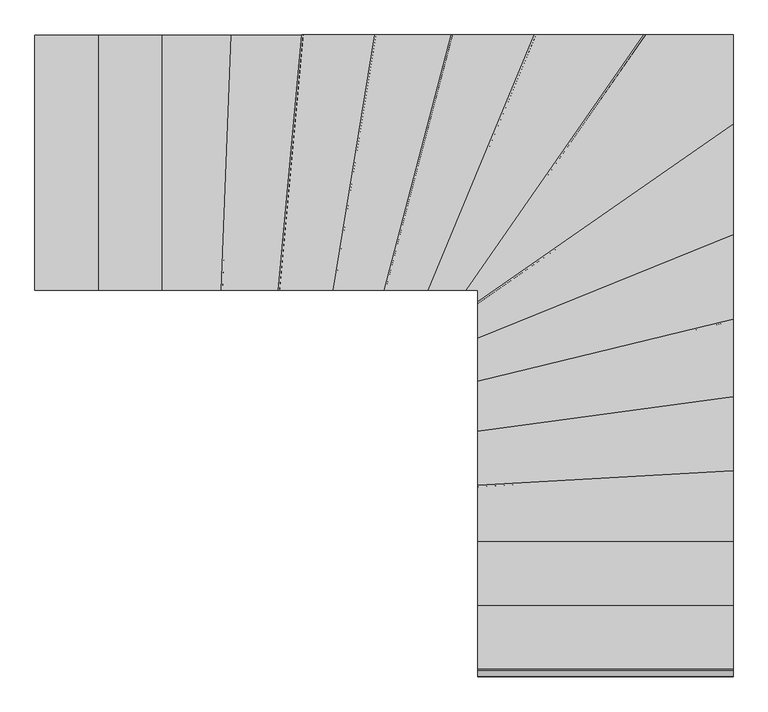
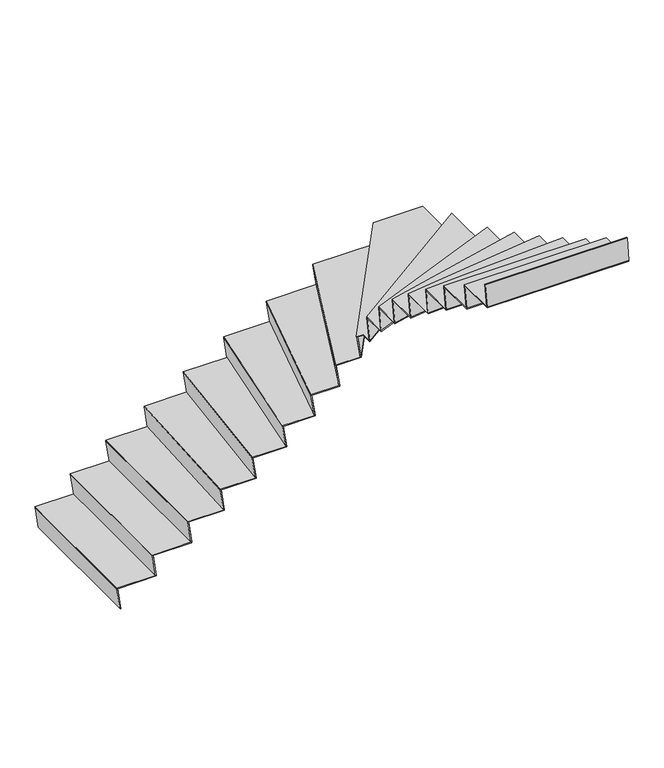
"""IFC4 building model written with IfcOpenShell, lengths in millimetres: stair flight geometry."""

from ifc_helpers import new_model, si_unit, origin, place, context, project, spatial, faceted_brep, source, transform, mapped, element, save


def stair_flight_e103a2b8(model_context):
    return source(origin(), model_context, "Body", "Brep", [
        faceted_brep([(2065.7472679, 3026.6218979, 176.4705882), (2066.5972679, 3026.6218979, 170.4705882), (2066.5972679, 4126.6218979, 170.4705882), (2065.7472679, 4126.6218979, 176.4705882), (1759.6873587, 4126.6218979, 176.4705882), (1759.6873587, 3026.6218979, 176.4705882), (1760.5373587, 3026.6218979, 170.4705882), (1760.5373587, 4126.6218979, 170.4705882)], [[[0, 1, 2, 3]], [[3, 4, 5, 0]], [[2, 1, 6, 7]], [[4, 3, 2, 7]], [[0, 5, 6, 1]], [[5, 4, 7, 6]]]),
        faceted_brep([(1760.5373587, 3026.6218979, 170.4705882), (1784.6873587, 3026.6218979, 0.0), (1790.7472679, 3026.6218979, 0.0), (1766.5972679, 3026.6218979, 170.4705882), (1760.5373587, 4126.6218979, 170.4705882), (1766.5972679, 4126.6218979, 170.4705882), (1790.7472679, 4126.6218979, 0.0), (1784.6873587, 4126.6218979, 0.0)], [[[0, 1, 2, 3]], [[4, 5, 6, 7]], [[1, 0, 4, 7]], [[2, 1, 7, 6]], [[3, 2, 6, 5]], [[0, 3, 5, 4]]]),
        faceted_brep([(2035.5373587, 3026.6218979, 346.9411765), (2059.6873587, 3026.6218979, 176.4705882), (2065.7472679, 3026.6218979, 176.4705882), (2041.5972679, 3026.6218979, 346.9411765), (2035.5373587, 4126.6218979, 346.9411765), (2041.5972679, 4126.6218979, 346.9411765), (2065.7472679, 4126.6218979, 176.4705882), (2059.6873587, 4126.6218979, 176.4705882)], [[[0, 1, 2, 3]], [[4, 5, 6, 7]], [[1, 0, 4, 7]], [[2, 1, 7, 6]], [[3, 2, 6, 5]], [[0, 3, 5, 4]]]),
        faceted_brep([(2340.7472679, 4126.6218979, 352.9411765), (2034.6873587, 4126.6218979, 352.9411765), (2034.6873587, 3026.6218979, 352.9411765), (2340.7472679, 3026.6218979, 352.9411765), (2341.5972679, 4126.6218979, 346.9411765), (2341.5972679, 3026.6218979, 346.9411765), (2035.5373587, 3026.6218979, 346.9411765), (2035.5373587, 4126.6218979, 346.9411765)], [[[0, 1, 2, 3]], [[4, 5, 6, 7]], [[1, 0, 4, 7]], [[3, 2, 6, 5]], [[3, 5, 4, 0]], [[2, 1, 7, 6]]]),
        faceted_brep([(2310.5373587, 3026.6218979, 523.4117647), (2334.6873587, 3026.6218979, 352.9411765), (2340.7472679, 3026.6218979, 352.9411765), (2316.5972679, 3026.6218979, 523.4117647), (2310.5373587, 4126.6218979, 523.4117647), (2316.5972679, 4126.6218979, 523.4117647), (2340.7472679, 4126.6218979, 352.9411765), (2334.6873587, 4126.6218979, 352.9411765)], [[[0, 1, 2, 3]], [[4, 5, 6, 7]], [[1, 0, 4, 7]], [[2, 1, 7, 6]], [[3, 2, 6, 5]], [[0, 3, 5, 4]]]),
        faceted_brep([(2637.9370393, 4126.6218979, 529.4117647), (2309.6873587, 4126.6218979, 529.4117647), (2309.6873587, 3026.6218979, 529.4117647), (2593.6079182, 3026.6218979, 529.4117647), (2638.7877292, 4126.6218979, 523.4117647), (2594.4586082, 3026.6218979, 523.4117647), (2310.5373587, 3026.6218979, 523.4117647), (2310.5373587, 4126.6218979, 523.4117647)], [[[0, 1, 2, 3]], [[4, 5, 6, 7]], [[1, 0, 4, 7]], [[3, 2, 6, 5]], [[3, 5, 4, 0]], [[2, 1, 7, 6]]]),
        faceted_brep([(2563.3734881, 3026.6218979, 699.8823529), (2587.5430903, 3026.6218979, 529.4117647), (2593.6079182, 3026.6218979, 529.4117647), (2569.4383161, 3026.6218979, 699.8823529), (2607.7026092, 4126.6218979, 699.8823529), (2613.7674371, 4126.6218979, 699.8823529), (2637.9370393, 4126.6218979, 529.4117647), (2631.8722113, 4126.6218979, 529.4117647)], [[[0, 1, 2, 3]], [[4, 5, 6, 7]], [[1, 0, 4, 7]], [[2, 1, 7, 6]], [[3, 2, 6, 5]], [[0, 3, 5, 4]]]),
        faceted_brep([(2941.764971, 4126.6218979, 705.8823529), (2606.8519192, 4126.6218979, 705.8823529), (2562.5227982, 3026.6218979, 705.8823529), (2839.9948598, 3026.6218979, 705.8823529), (2942.6186011, 4126.6218979, 699.8823529), (2840.8484899, 3026.6218979, 699.8823529), (2563.3734881, 3026.6218979, 699.8823529), (2607.7026092, 4126.6218979, 699.8823529)], [[[0, 1, 2, 3]], [[4, 5, 6, 7]], [[1, 0, 4, 7]], [[3, 2, 6, 5]], [[3, 5, 4, 0]], [[2, 1, 7, 6]]]),
        faceted_brep([(2809.6559332, 3026.6218979, 876.3529412), (2833.9090705, 3026.6218979, 705.8823529), (2839.9948598, 3026.6218979, 705.8823529), (2815.7417225, 3026.6218979, 876.3529412), (2911.4260444, 4126.6218979, 876.3529412), (2917.5118337, 4126.6218979, 876.3529412), (2941.764971, 4126.6218979, 705.8823529), (2935.6791818, 4126.6218979, 705.8823529)], [[[0, 1, 2, 3]], [[4, 5, 6, 7]], [[1, 0, 4, 7]], [[2, 1, 7, 6]], [[3, 2, 6, 5]], [[0, 3, 5, 4]]]),
        faceted_brep([(3255.7315376, 4126.6218979, 882.3529412), (2910.5724143, 4126.6218979, 882.3529412), (2808.8023031, 3026.6218979, 882.3529412), (3076.5814578, 3026.6218979, 882.3529412), (3256.5927368, 4126.6218979, 876.3529412), (3077.442657, 3026.6218979, 876.3529412), (2809.6559332, 3026.6218979, 876.3529412), (2911.4260444, 4126.6218979, 876.3529412)], [[[0, 1, 2, 3]], [[4, 5, 6, 7]], [[1, 0, 4, 7]], [[3, 2, 6, 5]], [[3, 5, 4, 0]], [[2, 1, 7, 6]]]),
        faceted_brep([(3045.973518, 3026.6218979, 1052.8235294), (3070.4417062, 3026.6218979, 882.3529412), (3076.5814578, 3026.6218979, 882.3529412), (3052.1132695, 3026.6218979, 1052.8235294), (3225.1235978, 4126.6218979, 1052.8235294), (3231.2633493, 4126.6218979, 1052.8235294), (3255.7315376, 4126.6218979, 882.3529412), (3249.591786, 4126.6218979, 882.3529412)], [[[0, 1, 2, 3]], [[4, 5, 6, 7]], [[1, 0, 4, 7]], [[2, 1, 7, 6]], [[3, 2, 6, 5]], [[0, 3, 5, 4]]]),
        faceted_brep([(3586.3171605, 4126.6218979, 1058.8235294), (3224.2623986, 4126.6218979, 1058.8235294), (3045.1123188, 3026.6218979, 1058.8235294), (3297.2859801, 3026.6218979, 1058.8235294), (3587.196013, 4126.6218979, 1052.8235294), (3298.1648327, 3026.6218979, 1052.8235294), (3045.973518, 3026.6218979, 1052.8235294), (3225.1235978, 4126.6218979, 1052.8235294)], [[[0, 1, 2, 3]], [[4, 5, 6, 7]], [[1, 0, 4, 7]], [[3, 2, 6, 5]], [[3, 5, 4, 0]], [[2, 1, 7, 6]]]),
        faceted_brep([(3266.0506211, 3026.6218979, 1229.2941176), (3291.0203724, 3026.6218979, 1058.8235294), (3297.2859801, 3026.6218979, 1058.8235294), (3272.3162288, 3026.6218979, 1229.2941176), (3555.0818014, 4126.6218979, 1229.2941176), (3561.3474091, 4126.6218979, 1229.2941176), (3586.3171605, 4126.6218979, 1058.8235294), (3580.0515527, 4126.6218979, 1058.8235294)], [[[0, 1, 2, 3]], [[4, 5, 6, 7]], [[1, 0, 4, 7]], [[2, 1, 7, 6]], [[3, 2, 6, 5]], [[0, 3, 5, 4]]]),
        faceted_brep([(3947.0915643, 4126.6218979, 1235.2941176), (3554.2029489, 4126.6218979, 1235.2941176), (3265.1717685, 3026.6218979, 1235.2941176), (3489.7295318, 3026.6218979, 1235.2941176), (3948.0121092, 4126.6218979, 1229.2941176), (3490.6500767, 3026.6218979, 1229.2941176), (3266.0506211, 3026.6218979, 1229.2941176), (3555.0818014, 4126.6218979, 1229.2941176)], [[[0, 1, 2, 3]], [[4, 5, 6, 7]], [[1, 0, 4, 7]], [[3, 2, 6, 5]], [[3, 5, 4, 0]], [[2, 1, 7, 6]]]),
        faceted_brep([(3457.0123806, 3026.6218979, 1405.7647059), (3483.1666863, 3026.6218979, 1235.2941176), (3489.7295318, 3026.6218979, 1235.2941176), (3463.5752261, 3026.6218979, 1405.7647059), (3914.3744131, 4126.6218979, 1405.7647059), (3920.9372586, 4126.6218979, 1405.7647059), (3947.0915643, 4126.6218979, 1235.2941176), (3940.5287188, 4126.6218979, 1235.2941176)], [[[0, 1, 2, 3]], [[4, 5, 6, 7]], [[1, 0, 4, 7]], [[2, 1, 7, 6]], [[3, 2, 6, 5]], [[0, 3, 5, 4]]]),
        faceted_brep([(4423.3254739, 4126.6218979, 1411.7647059), (3913.4538681, 4126.6218979, 1411.7647059), (3456.0918357, 3026.6218979, 1411.7647059), (3656.5915421, 3026.6218979, 1411.7647059), (4424.3615859, 4126.6218979, 1405.7647059), (3657.6276541, 3026.6218979, 1405.7647059), (3457.0123806, 3026.6218979, 1405.7647059), (3914.3744131, 4126.6218979, 1405.7647059)], [[[0, 1, 2, 3]], [[4, 5, 6, 7]], [[1, 0, 4, 7]], [[3, 2, 6, 5]], [[3, 5, 4, 0]], [[2, 1, 7, 6]]]),
        faceted_brep([(3619.7670134, 3026.6218979, 1582.2352941), (3649.2047837, 3026.6218979, 1411.7647059), (3656.5915421, 3026.6218979, 1411.7647059), (3627.1537718, 3026.6218979, 1582.2352941), (4386.5009452, 4126.6218979, 1582.2352941), (4393.8877036, 4126.6218979, 1582.2352941), (4423.3254739, 4126.6218979, 1411.7647059), (4415.9387155, 4126.6218979, 1411.7647059)], [[[0, 1, 2, 3]], [[4, 5, 6, 7]], [[1, 0, 4, 7]], [[2, 1, 7, 6]], [[3, 2, 6, 5]], [[0, 3, 5, 4]]]),
        faceted_brep([(4769.6425896, 3704.5835008, 1588.2352941), (4769.6425896, 4126.6218979, 1588.2352941), (4385.4648332, 4126.6218979, 1588.2352941), (3618.7309014, 3026.6218979, 1588.2352941), (3669.6425896, 3026.6218979, 1588.2352941), (3669.6425896, 2937.849569, 1588.2352941), (4769.6425896, 3703.5473888, 1582.2352941), (3669.6425896, 2936.813457, 1582.2352941), (3669.6425896, 3026.6218979, 1582.2352941), (3619.7670134, 3026.6218979, 1582.2352941), (4386.5009452, 4126.6218979, 1582.2352941), (4769.6425896, 4126.6218979, 1582.2352941)], [[[0, 1, 2, 3, 4, 5]], [[6, 7, 8, 9, 10, 11]], [[1, 0, 6, 11]], [[2, 1, 11, 10]], [[4, 3, 9, 8]], [[5, 4, 8, 7]], [[5, 7, 6, 0]], [[3, 2, 10, 9]]]),
        faceted_brep([(3669.6425896, 2974.6740977, 1758.7058824), (3669.6425896, 2945.2363274, 1588.2352941), (3669.6425896, 2937.849569, 1588.2352941), (3669.6425896, 2967.2873392, 1758.7058824), (4769.6425896, 3741.4080295, 1758.7058824), (4769.6425896, 3734.0212711, 1758.7058824), (4769.6425896, 3704.5835008, 1588.2352941), (4769.6425896, 3711.9702592, 1588.2352941)], [[[0, 1, 2, 3]], [[4, 5, 6, 7]], [[1, 0, 4, 7]], [[2, 1, 7, 6]], [[3, 2, 6, 5]], [[0, 3, 5, 4]]]),
        faceted_brep([(4769.6425896, 3231.5060834, 1764.7058824), (4769.6425896, 3742.4441415, 1764.7058824), (3669.6425896, 2975.7102097, 1764.7058824), (3669.6425896, 2784.9507322, 1764.7058824), (4769.6425896, 3230.5887121, 1758.7058824), (3669.6425896, 2784.0333608, 1758.7058824), (3669.6425896, 2974.6740977, 1758.7058824), (4769.6425896, 3741.4080295, 1758.7058824)], [[[0, 1, 2, 3]], [[4, 5, 6, 7]], [[1, 0, 4, 7]], [[3, 2, 6, 5]], [[3, 5, 4, 0]], [[2, 1, 7, 6]]]),
        faceted_brep([(3669.6425896, 2817.5550913, 1935.1764706), (3669.6425896, 2791.4909523, 1764.7058824), (3669.6425896, 2784.9507322, 1764.7058824), (3669.6425896, 2811.0148712, 1935.1764706), (4769.6425896, 3264.1104426, 1935.1764706), (4769.6425896, 3257.5702224, 1935.1764706), (4769.6425896, 3231.5060834, 1764.7058824), (4769.6425896, 3238.0463036, 1764.7058824)], [[[0, 1, 2, 3]], [[4, 5, 6, 7]], [[1, 0, 4, 7]], [[2, 1, 7, 6]], [[3, 2, 6, 5]], [[0, 3, 5, 4]]]),
        faceted_brep([(4769.6425896, 2868.6989632, 1941.1764706), (4769.6425896, 3265.027814, 1941.1764706), (3669.6425896, 2818.4724627, 1941.1764706), (3669.6425896, 2600.6974331, 1941.1764706), (4769.6425896, 2867.8240992, 1935.1764706), (3669.6425896, 2599.8225691, 1935.1764706), (3669.6425896, 2817.5550913, 1935.1764706), (4769.6425896, 3264.1104426, 1935.1764706)], [[[0, 1, 2, 3]], [[4, 5, 6, 7]], [[1, 0, 4, 7]], [[3, 2, 6, 5]], [[3, 5, 4, 0]], [[2, 1, 7, 6]]]),
        faceted_brep([(3669.6425896, 2631.7910379, 2111.6470588), (3669.6425896, 2606.9346059, 1941.1764706), (3669.6425896, 2600.6974331, 1941.1764706), (3669.6425896, 2625.5538651, 2111.6470588), (4769.6425896, 2899.792568, 2111.6470588), (4769.6425896, 2893.5553952, 2111.6470588), (4769.6425896, 2868.6989632, 1941.1764706), (4769.6425896, 2874.936136, 1941.1764706)], [[[0, 1, 2, 3]], [[4, 5, 6, 7]], [[1, 0, 4, 7]], [[2, 1, 7, 6]], [[3, 2, 6, 5]], [[0, 3, 5, 4]]]),
        faceted_brep([(4769.6425896, 2534.7846987, 2117.6470588), (4769.6425896, 2900.667432, 2117.6470588), (3669.6425896, 2632.665902, 2117.6470588), (3669.6425896, 2385.8621086, 2117.6470588), (4769.6425896, 2533.9269443, 2111.6470588), (3669.6425896, 2385.0043542, 2111.6470588), (3669.6425896, 2631.7910379, 2111.6470588), (4769.6425896, 2899.792568, 2111.6470588)], [[[0, 1, 2, 3]], [[4, 5, 6, 7]], [[1, 0, 4, 7]], [[3, 2, 6, 5]], [[3, 5, 4, 0]], [[2, 1, 7, 6]]]),
        faceted_brep([(3669.6425896, 2416.3476175, 2288.1176471), (3669.6425896, 2391.9773013, 2117.6470588), (3669.6425896, 2385.8621086, 2117.6470588), (3669.6425896, 2410.2324248, 2288.1176471), (4769.6425896, 2565.2702077, 2288.1176471), (4769.6425896, 2559.1550149, 2288.1176471), (4769.6425896, 2534.7846987, 2117.6470588), (4769.6425896, 2540.8998915, 2117.6470588)], [[[0, 1, 2, 3]], [[4, 5, 6, 7]], [[1, 0, 4, 7]], [[2, 1, 7, 6]], [[3, 2, 6, 5]], [[0, 3, 5, 4]]]),
        faceted_brep([(4769.6425896, 2217.471517, 2294.1176471), (4769.6425896, 2566.1279621, 2294.1176471), (3669.6425896, 2417.2053719, 2294.1176471), (3669.6425896, 2153.6374895, 2294.1176471), (4769.6425896, 2216.6200869, 2288.1176471), (3669.6425896, 2152.7860594, 2288.1176471), (3669.6425896, 2416.3476175, 2288.1176471), (4769.6425896, 2565.2702077, 2288.1176471)], [[[0, 1, 2, 3]], [[4, 5, 6, 7]], [[1, 0, 4, 7]], [[3, 2, 6, 5]], [[3, 5, 4, 0]], [[2, 1, 7, 6]]]),
        faceted_brep([(3669.6425896, 2183.8982232, 2464.5882353), (3669.6425896, 2159.7075938, 2294.1176471), (3669.6425896, 2153.6374895, 2294.1176471), (3669.6425896, 2177.8281189, 2464.5882353), (4769.6425896, 2247.7322507, 2464.5882353), (4769.6425896, 2241.6621464, 2464.5882353), (4769.6425896, 2217.471517, 2294.1176471), (4769.6425896, 2223.5416213, 2294.1176471)], [[[0, 1, 2, 3]], [[4, 5, 6, 7]], [[1, 0, 4, 7]], [[2, 1, 7, 6]], [[3, 2, 6, 5]], [[0, 3, 5, 4]]]),
        faceted_brep([(4769.6425896, 1910.6067578, 2470.5882353), (4769.6425896, 2248.5836807, 2470.5882353), (3669.6425896, 2184.7496533, 2470.5882353), (3669.6425896, 1910.6067578, 2470.5882353), (4769.6425896, 1909.7567578, 2464.5882353), (3669.6425896, 1909.7567578, 2464.5882353), (3669.6425896, 2183.8982232, 2464.5882353), (4769.6425896, 2247.7322507, 2464.5882353)], [[[0, 1, 2, 3]], [[4, 5, 6, 7]], [[1, 0, 4, 7]], [[3, 2, 6, 5]], [[3, 5, 4, 0]], [[2, 1, 7, 6]]]),
        faceted_brep([(3669.6425896, 1940.816667, 2641.0588235), (3669.6425896, 1916.666667, 2470.5882353), (3669.6425896, 1910.6067578, 2470.5882353), (3669.6425896, 1934.7567578, 2641.0588235), (4769.6425896, 1940.816667, 2641.0588235), (4769.6425896, 1934.7567578, 2641.0588235), (4769.6425896, 1910.6067578, 2470.5882353), (4769.6425896, 1916.666667, 2470.5882353)], [[[0, 1, 2, 3]], [[4, 5, 6, 7]], [[1, 0, 4, 7]], [[2, 1, 7, 6]], [[3, 2, 6, 5]], [[0, 3, 5, 4]]]),
        faceted_brep([(4769.6425896, 1635.6067578, 2647.0588235), (4769.6425896, 1941.666667, 2647.0588235), (3669.6425896, 1941.666667, 2647.0588235), (3669.6425896, 1635.6067578, 2647.0588235), (4769.6425896, 1634.7567578, 2641.0588235), (3669.6425896, 1634.7567578, 2641.0588235), (3669.6425896, 1940.816667, 2641.0588235), (4769.6425896, 1940.816667, 2641.0588235)], [[[0, 1, 2, 3]], [[4, 5, 6, 7]], [[1, 0, 4, 7]], [[3, 2, 6, 5]], [[3, 5, 4, 0]], [[2, 1, 7, 6]]]),
        faceted_brep([(3669.6425896, 1665.816667, 2817.5294118), (3669.6425896, 1641.666667, 2647.0588235), (3669.6425896, 1635.6067578, 2647.0588235), (3669.6425896, 1659.7567578, 2817.5294118), (4769.6425896, 1665.816667, 2817.5294118), (4769.6425896, 1659.7567578, 2817.5294118), (4769.6425896, 1635.6067578, 2647.0588235), (4769.6425896, 1641.666667, 2647.0588235)], [[[0, 1, 2, 3]], [[4, 5, 6, 7]], [[1, 0, 4, 7]], [[2, 1, 7, 6]], [[3, 2, 6, 5]], [[0, 3, 5, 4]]]),
        faceted_brep([(3669.6425896, 1390.816667, 2994.0), (3669.6425896, 1366.666667, 2823.5294118), (3669.6425896, 1360.6067578, 2823.5294118), (3669.6425896, 1384.7567578, 2994.0), (4769.6425896, 1390.816667, 2994.0), (4769.6425896, 1384.7567578, 2994.0), (4769.6425896, 1360.6067578, 2823.5294118), (4769.6425896, 1366.666667, 2823.5294118)], [[[0, 1, 2, 3]], [[4, 5, 6, 7]], [[1, 0, 4, 7]], [[2, 1, 7, 6]], [[3, 2, 6, 5]], [[0, 3, 5, 4]]]),
        faceted_brep([(4769.6425896, 1360.6067578, 2823.5294118), (4769.6425896, 1666.666667, 2823.5294118), (3669.6425896, 1666.666667, 2823.5294118), (3669.6425896, 1360.6067578, 2823.5294118), (4769.6425896, 1359.7567578, 2817.5294118), (3669.6425896, 1359.7567578, 2817.5294118), (3669.6425896, 1665.816667, 2817.5294118), (4769.6425896, 1665.816667, 2817.5294118)], [[[0, 1, 2, 3]], [[4, 5, 6, 7]], [[1, 0, 4, 7]], [[3, 2, 6, 5]], [[3, 5, 4, 0]], [[2, 1, 7, 6]]]),
    ])


if __name__ == "__main__":
    model = new_model("IFC4")
    model_context = context("Model", 3, world=origin())
    ifc_project = project(units=[si_unit("LENGTHUNIT", "METRE", prefix="MILLI")], contexts=[model_context])
    site = spatial("IfcSite", under=ifc_project)
    building = spatial("IfcBuilding", under=site)
    placement = place(None, origin())
    stair_flight_shape = stair_flight_e103a2b8(model_context)
    element("IfcStairFlight", 1, at=placement, inside=building, context=model_context, shape_type="MappedRepresentation", body=[
        mapped(stair_flight_shape, transform((0.0, 0.0, 0.0), x_axis=(1.0, 0.0, 0.0), y_axis=(0.0, 1.0, 0.0), z_axis=(0.0, 0.0, 1.0))),
    ])
    save(model, "model.ifc")

# Revit data of these elements
# Element 1 (IfcStairFlight)
#   Materials on its faces: "Acero, acabado de pintura, gris oscuro"
# Materials
#   "Acero, acabado de pintura, gris oscuro": class "Metal", colour RGB 89 89 89, transparency 0, Description = "Acero, acabado de pintura, gris oscuro, brillante", Cost = 0
